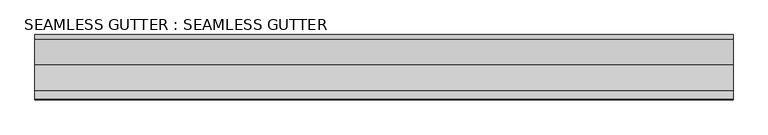
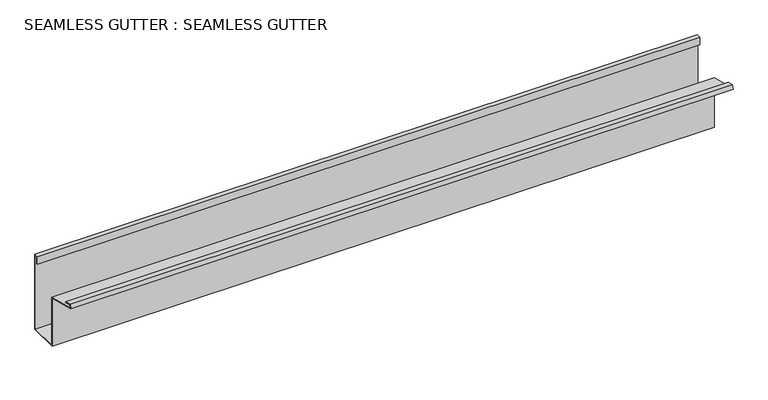
"""IFC4 building model written with IfcOpenShell, lengths in millimetres: proxy geometry, SEAMLESS GUTTER : SEAMLESS GUTTER."""

from ifc_helpers import new_model, si_unit, frame, origin, place, context, project, spatial, polyline, outline, extrude, source, transform, mapped, element, save


def seamless_gutter_seamless_gutter_9d60836d(model_context):
    return source(origin(), model_context, "Body", "SweptSolid", [
        extrude(outline(polyline([(4442.9441527, 41585.7855856), (4455.6441528, 41585.7855856), (4455.6441528, 41345.9729908), (4365.6886967, 41345.9729908), (4365.6886967, 41500.4350951), (4268.4140616, 41525.5769203), (4271.5920979, 41537.8728581), (4294.6469812, 41531.9140401), (4294.0510994, 41529.6085518), (4273.3017044, 41534.971488), (4271.3154317, 41527.2865268), (4368.0699467, 41502.2791331), (4368.0699467, 41348.3542408), (4453.2629028, 41348.3542408), (4453.2629028, 41583.4043356), (4445.3254027, 41583.4043356), (4445.3254027, 41561.9730856), (4442.9441527, 41561.9730856), (4442.9441527, 41585.7855856)])), frame((255.0171875, 0.0, 0.0), z_axis=(1.0, 0.0, 0.0), x_axis=(0.0, 1.0, 0.0)), (0.0, 0.0, 1.0), 1999.85),
    ])


if __name__ == "__main__":
    model = new_model("IFC4")
    model_context = context("Model", 3, world=origin())
    ifc_project = project(units=[si_unit("LENGTHUNIT", "METRE", prefix="MILLI")], contexts=[model_context])
    site = spatial("IfcSite", under=ifc_project)
    building = spatial("IfcBuilding", under=site)
    placement = place(None, origin())
    seamless_gutter_seamless_gutter_shape = seamless_gutter_seamless_gutter_9d60836d(model_context)
    element("IfcBuildingElementProxy", 1, Name="SEAMLESS GUTTER : SEAMLESS GUTTER", ObjectType="SEAMLESS GUTTER : SEAMLESS GUTTER", at=placement, inside=building, context=model_context, shape_type="MappedRepresentation", body=[
        mapped(seamless_gutter_seamless_gutter_shape, transform((0.0, 0.0, 0.0), x_axis=(1.0, 0.0, 0.0), y_axis=(0.0, 1.0, 0.0), z_axis=(0.0, 0.0, 1.0))),
    ])
    save(model, "model.ifc")

# Revit data of these elements
# Type "SEAMLESS GUTTER : SEAMLESS GUTTER"
#   NameOverride = "SEAMLESS GUTTER"
# Element 1 (IfcBuildingElementProxy, "SEAMLESS GUTTER : SEAMLESS GUTTER")
#   Materials on its faces: "CONT. SEAMLESS 16 GA COPPER BRAKE METAL GUTTER"
# Materials
#   "CONT. SEAMLESS 16 GA COPPER BRAKE METAL GUTTER": class "Unassigned", colour RGB 128 128 128, transparency 0
